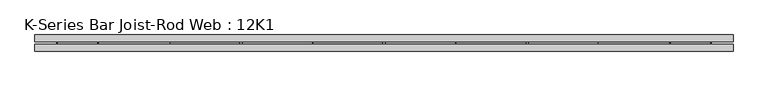
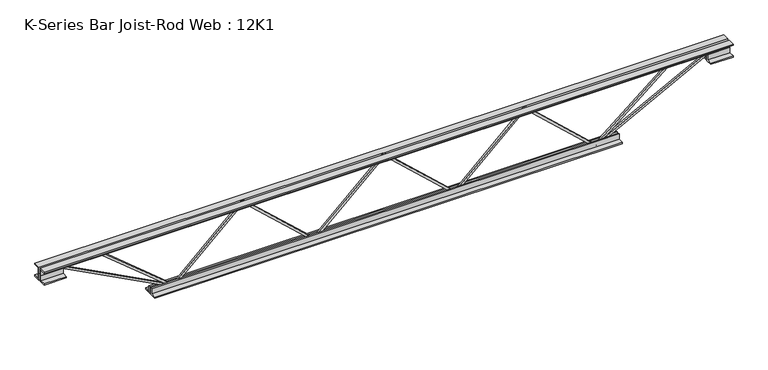
"""IFC4 building model written with IfcOpenShell, lengths in millimetres: beam geometry, K-Series Bar Joist-Rod Web : 12K1."""

from ifc_helpers import new_model, si_unit, frame, origin, place, context, project, spatial, polyline, outline, extrude, source, transform, mapped, element, save


def k_series_bar_joist_rod_web_12k1_4b334fa5(model_context):
    return source(origin(), model_context, "Body", "SweptSolid", [
        extrude(outline(polyline([(-141.2875, -323.3208333), (-150.8125, -323.3208333), (-150.8125, -318.2860584), (141.2875, -1.3152251), (141.2875, 1.3152251), (-150.8125, 318.2860584), (-150.8125, 323.3208333), (-141.2875, 323.3208333), (-141.2875, 322.0056082), (150.8125, 5.0347749), (150.8125, -5.0347749), (-141.2875, -322.0056082), (-141.2875, -323.3208333)])), frame((0.0, -4.7625, 0.0), z_axis=(0.0, 1.0, 0.0), x_axis=(0.0, 0.0, 1.0)), (0.0, 0.0, 1.0), 9.525),
        extrude(outline(polyline([(-141.2875, 323.3208333), (-150.8125, 323.3208333), (-150.8125, 328.3556082), (141.2875, 645.3264416), (141.2875, 647.9568918), (-150.8125, 964.9277251), (-150.8125, 969.9625), (-141.2875, 969.9625), (-141.2875, 968.6472749), (150.8125, 651.6764416), (150.8125, 641.6068918), (-141.2875, 324.6360584), (-141.2875, 323.3208333)])), frame((0.0, -4.7625, 0.0), z_axis=(0.0, 1.0, 0.0), x_axis=(0.0, 0.0, 1.0)), (0.0, 0.0, 1.0), 9.525),
        extrude(outline(polyline([(-141.2875, -969.9625), (-150.8125, -969.9625), (-150.8125, -964.9277251), (141.2875, -647.9568918), (141.2875, -645.3264416), (-150.8125, -328.3556082), (-150.8125, -323.3208333), (-141.2875, -323.3208333), (-141.2875, -324.6360584), (150.8125, -641.6068918), (150.8125, -651.6764416), (-141.2875, -968.6472749), (-141.2875, -969.9625)])), frame((0.0, -4.7625, 0.0), z_axis=(0.0, 1.0, 0.0), x_axis=(0.0, 0.0, 1.0)), (0.0, 0.0, 1.0), 9.525),
        extrude(outline(polyline([(4.7625, 152.4), (36.5125, 152.4), (36.5125, 146.05), (11.1125, 146.05), (11.1125, 120.65), (4.7625, 120.65), (4.7625, 152.4)])), frame((-1579.5625, 0.0, 0.0), z_axis=(1.0, 0.0, 0.0), x_axis=(0.0, 1.0, 0.0)), (0.0, 0.0, 1.0), 3159.125),
        extrude(outline(polyline([(-4.7625, 152.4), (-4.7625, 120.65), (-11.1125, 120.65), (-11.1125, 146.05), (-36.5125, 146.05), (-36.5125, 152.4), (-4.7625, 152.4)])), frame((-1579.5625, 0.0, 0.0), z_axis=(1.0, 0.0, 0.0), x_axis=(0.0, 1.0, 0.0)), (0.0, 0.0, 1.0), 3159.125),
        extrude(outline(polyline([(-4.7625, 88.9), (-36.5125, 88.9), (-36.5125, 95.25), (-11.1125, 95.25), (-11.1125, 120.65), (-4.7625, 120.65), (-4.7625, 88.9)])), frame((-1579.5625, 0.0, 0.0), z_axis=(1.0, 0.0, 0.0), x_axis=(0.0, 1.0, 0.0)), (0.0, 0.0, 1.0), 101.6),
        extrude(outline(polyline([(36.5125, 88.9), (4.7625, 88.9), (4.7625, 120.65), (11.1125, 120.65), (11.1125, 95.25), (36.5125, 95.25), (36.5125, 88.9)])), frame((-1579.5625, 0.0, 0.0), z_axis=(1.0, 0.0, 0.0), x_axis=(0.0, 1.0, 0.0)), (0.0, 0.0, 1.0), 101.6),
        extrude(outline(polyline([(4.7625, 88.9), (4.7625, 120.65), (11.1125, 120.65), (11.1125, 95.25), (36.5125, 95.25), (36.5125, 88.9), (4.7625, 88.9)])), frame((1477.9625, 0.0, 0.0), z_axis=(1.0, 0.0, 0.0), x_axis=(0.0, 1.0, 0.0)), (0.0, 0.0, 1.0), 101.6),
        extrude(outline(polyline([(-4.7625, 88.9), (-36.5125, 88.9), (-36.5125, 95.25), (-11.1125, 95.25), (-11.1125, 120.65), (-4.7625, 120.65), (-4.7625, 88.9)])), frame((1477.9625, 0.0, 0.0), z_axis=(1.0, 0.0, 0.0), x_axis=(0.0, 1.0, 0.0)), (0.0, 0.0, 1.0), 101.6),
        extrude(outline(polyline([(4.7625, -152.4), (4.7625, -120.65), (11.1125, -120.65), (11.1125, -146.05), (36.5125, -146.05), (36.5125, -152.4), (4.7625, -152.4)])), frame((-1071.5625, 0.0, 0.0), z_axis=(1.0, 0.0, 0.0), x_axis=(0.0, 1.0, 0.0)), (0.0, 0.0, 1.0), 2143.125),
        extrude(outline(polyline([(-4.7625, -152.4), (-36.5125, -152.4), (-36.5125, -146.05), (-11.1125, -146.05), (-11.1125, -120.65), (-4.7625, -120.65), (-4.7625, -152.4)])), frame((-1071.5625, 0.0, 0.0), z_axis=(1.0, 0.0, 0.0), x_axis=(0.0, 1.0, 0.0)), (0.0, 0.0, 1.0), 2143.125),
        extrude(outline(polyline([(0.0, -9.525), (0.0, 0.0), (573.7533355, 0.0), (573.7533355, -9.525), (0.0, -9.525)])), frame((-1480.1762714, 4.7625, 116.4332925), z_axis=(0.46483389898951427, 0.0, 0.8853979028381568), x_axis=(0.8853979028381568, 0.0, -0.46483389898951427)), (0.0, 0.0, 1.0), 9.525),
        extrude(outline(polyline([(0.0, -9.525), (0.0, 0.0), (419.1243864, 0.0), (419.1243864, -9.525), (0.0, -9.525)])), frame((-1296.3138388, 4.7625, 116.9761134), z_axis=(0.6363266100943057, 0.0, 0.7714197594603663), x_axis=(0.7714197594603663, 0.0, -0.6363266100943057)), (0.0, 0.0, 1.0), 9.525),
        extrude(outline(polyline([(0.0, -9.525), (0.0, 0.0), (573.7533355, 0.0), (573.7533355, -9.525), (0.0, -9.525)])), frame((1480.1762714, -4.7625, 116.4332925), z_axis=(-0.4648338989894941, 0.0, 0.8853979028381673), x_axis=(-0.8853979028381673, 0.0, -0.4648338989894941)), (0.0, 0.0, 1.0), 9.525),
        extrude(outline(polyline([(0.0, -9.525), (0.0, 0.0), (419.1243864, 0.0), (419.1243864, -9.525), (0.0, -9.525)])), frame((1296.3138388, -4.7625, 116.9761134), z_axis=(-0.6363266100942991, 0.0, 0.7714197594603718), x_axis=(-0.7714197594603718, 0.0, -0.6363266100942991)), (0.0, 0.0, 1.0), 9.525),
    ])


if __name__ == "__main__":
    model = new_model("IFC4")
    model_context = context("Model", 3, world=origin())
    ifc_project = project(units=[si_unit("LENGTHUNIT", "METRE", prefix="MILLI")], contexts=[model_context])
    site = spatial("IfcSite", under=ifc_project)
    building = spatial("IfcBuilding", under=site)
    placement = place(None, origin())
    k_series_bar_joist_rod_web_12k1_shape = k_series_bar_joist_rod_web_12k1_4b334fa5(model_context)
    element("IfcBeam", 1, ObjectType="K-Series Bar Joist-Rod Web : 12K1", at=placement, inside=building, context=model_context, shape_type="MappedRepresentation", body=[
        mapped(k_series_bar_joist_rod_web_12k1_shape, transform((0.0, 0.0, 0.0), x_axis=(1.0, 0.0, 0.0), y_axis=(0.0, 1.0, 0.0), z_axis=(0.0, 0.0, 1.0))),
    ])
    save(model, "model.ifc")

# Revit data of these elements
# Type "K-Series Bar Joist-Rod Web : 12K1"
#   Assembly Code = "B1010350"
#   Wt = 5
#   Web Thickness = 0' - 0 3/8"
#   Start Offset [instance default] = 0' - 0"
#   Start Extension [instance default] = 0' - 0"
#   Seat Length = 0' - 4"
#   Seat Depth = 0' - 2 1/2"
#   PanelArrayLength [instance default] = 20' - 0"
#   Panel [instance default] = 2' - 0"
#   End Offset [instance default] = 0' - 0"
#   End Extension [instance default] = 0' - 0"
#   End Panel = 2' - 0"
#   Cord Leg = 0' - 1 1/4"
#   Chord Thickness = 0' - 0 1/4"
#   Length [instance default] = 24' - 0"
#   Depth = 1' - 0"
#   PanelArrayNum [instance default] = 10
#   Structural Material = none
# Element 1 (IfcBeam, "K-Series Bar Joist-Rod Web : 12K1")
#   PanelArrayLength = 6' - 4 3/8"
#   Panel = 2' - 1.45833"
#   PanelArrayNum = 3
